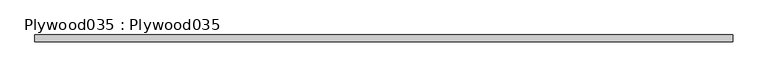
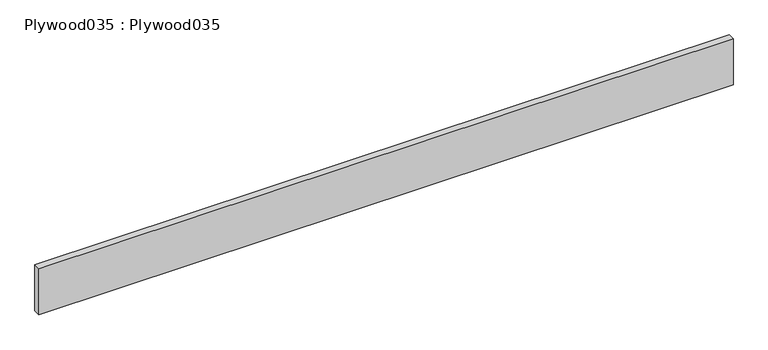
"""IFC4 building model written with IfcOpenShell, lengths in millimetres: proxy geometry, Plywood035 : Plywood035."""

from ifc_helpers import new_model, si_unit, frame, origin, place, context, project, spatial, polyline, outline, extrude, source, transform, mapped, element, save


def plywood035_plywood035_31689b76(model_context):
    return source(origin(), model_context, "Body", "SweptSolid", [
        extrude(outline(polyline([(14383.0178845, -5224.4032789), (14383.0178845, -5244.4501953), (12383.0178845, -5244.4501953), (12383.0178845, -5224.4032789), (14383.0178845, -5224.4032789)])), frame((0.0, 0.0, 42661.0807603), z_axis=(0.0, 0.0, 1.0), x_axis=(1.0, 0.0, 0.0)), (0.0, 0.0, 1.0), 139.7),
    ])


if __name__ == "__main__":
    model = new_model("IFC4")
    model_context = context("Model", 3, world=origin())
    ifc_project = project(units=[si_unit("LENGTHUNIT", "METRE", prefix="MILLI")], contexts=[model_context])
    site = spatial("IfcSite", under=ifc_project)
    building = spatial("IfcBuilding", under=site)
    placement = place(None, origin())
    plywood035_plywood035_shape = plywood035_plywood035_31689b76(model_context)
    element("IfcBuildingElementProxy", 1, Name="Plywood035 : Plywood035", ObjectType="Plywood035 : Plywood035", at=placement, inside=building, context=model_context, shape_type="MappedRepresentation", body=[
        mapped(plywood035_plywood035_shape, transform((0.0, 0.0, 0.0), x_axis=(1.0, 0.0, 0.0), y_axis=(0.0, 1.0, 0.0), z_axis=(0.0, 0.0, 1.0))),
    ])
    save(model, "model.ifc")

# Revit data of these elements
# Type "Plywood035 : Plywood035"
#   NameOverride = "Plywood035"
# Element 1 (IfcBuildingElementProxy, "Plywood035 : Plywood035")
#   Materials on its faces: "CDX PLYWOOD - SEE STRUCTURAL DWGS"
# Materials
#   "CDX PLYWOOD - SEE STRUCTURAL DWGS": class "Unassigned", colour RGB 177 130 114, transparency 0, Cost = 0
